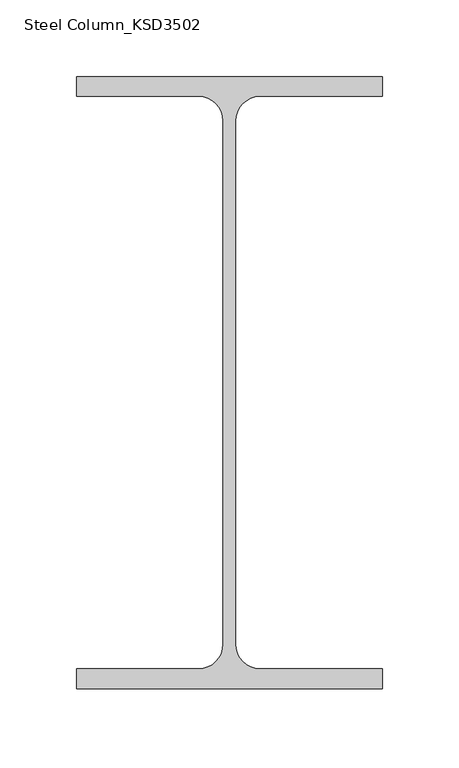
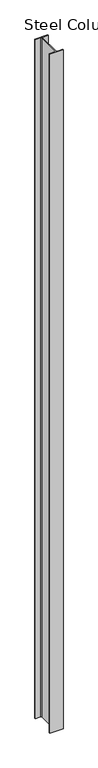
"""IFC4 building model written with IfcOpenShell, lengths in millimetres: column geometry, Steel Column_KSD3502 : H_SC_ASC_H-400×200x8x13."""

import ifcopenshell
import ifcopenshell.guid

model = None  # the IFC model being written
_history = None  # IfcOwnerHistory: only IFC2X3 demands one
_inside = {}  # id of a spatial element -> (the spatial element, [elements in it])
_under = {}  # id of a project, library or spatial element -> (it, [spatial elements below it])
_declared = {}  # id of a project -> (the project, [libraries it declares])
_typed = {}  # id of a type object -> (the type object, [elements of that type])
_made_of = {}  # id of a material, layer set ... -> (it, [elements and type objects made of it])


def new_model(schema):
    """Start an empty IFC model of exactly this schema.

    Asked for "IFC4X3", IfcOpenShell would pick the latest addendum, in which some entities
    have other attributes; the version numbers below select the first issue.
    IFC2X3 requires an IfcOwnerHistory on every rooted entity: one is made here for all.
    """
    global model, _history
    if schema == "IFC4X3":
        model = ifcopenshell.file(schema_version=(4, 3, 0, 0))
    else:
        model = ifcopenshell.file(schema=schema)
    _inside.clear()
    _under.clear()
    _declared.clear()
    _typed.clear()
    _made_of.clear()
    _history = None
    if model.schema == "IFC2X3":
        org = make("IfcOrganization", Name="unknown")
        user = make(
            "IfcPersonAndOrganization",
            ThePerson=make("IfcPerson", FamilyName="unknown"),
            TheOrganization=org,
        )
        app = make(
            "IfcApplication",
            ApplicationDeveloper=org,
            Version="unknown",
            ApplicationFullName="unknown",
            ApplicationIdentifier="unknown",
        )
        _history = make(
            "IfcOwnerHistory",
            OwningUser=user,
            OwningApplication=app,
            ChangeAction="ADDED",
            CreationDate=0,
        )
    return model


def make(cls, **values):
    """One entity of the class cls with the attributes given. An attribute that is None is left unset."""
    return model.create_entity(
        cls, **{name: value for name, value in values.items() if value is not None}
    )


def rooted(cls, **values):
    """An entity with a GlobalId (a new one), such as an element, a storey or a relation."""
    return make(cls, GlobalId=ifcopenshell.guid.new(), OwnerHistory=_history, **values)


def si_unit(unit_type, name, prefix=None):
    """IfcSIUnit, for example si_unit("LENGTHUNIT", "METRE", prefix="MILLI")."""
    return make("IfcSIUnit", UnitType=unit_type, Prefix=prefix, Name=name)


def assignment(units):
    """IfcUnitAssignment: the units of a project."""
    return None if units is None else make("IfcUnitAssignment", Units=units)


def point(xyz):
    """IfcCartesianPoint."""
    return None if xyz is None else make("IfcCartesianPoint", Coordinates=xyz)


def direction(xyz):
    """IfcDirection."""
    return None if xyz is None else make("IfcDirection", DirectionRatios=xyz)


def frame(location, z_axis=None, x_axis=None):
    """IfcAxis2Placement3D, a coordinate frame: its origin and axes. An axis left out is left unset."""
    return make(
        "IfcAxis2Placement3D",
        Location=point(location),
        Axis=direction(z_axis),
        RefDirection=direction(x_axis),
    )


def frame_2d(location, x_axis=None):
    """IfcAxis2Placement2D, a coordinate frame in the plane: its origin and x axis."""
    return make(
        "IfcAxis2Placement2D", Location=point(location), RefDirection=direction(x_axis)
    )


def origin():
    """The frame at (0, 0, 0) with its axes left unset."""
    return frame((0.0, 0.0, 0.0))


def place(relative_to, where):
    """IfcLocalPlacement: puts the frame where relative to a parent placement (None: the world)."""
    return make(
        "IfcLocalPlacement", PlacementRelTo=relative_to, RelativePlacement=where
    )


def context(
    kind, dimensions, precision=None, world=None, true_north=None, identifier=None
):
    """IfcGeometricRepresentationContext, for example the 3D "Model" context."""
    return make(
        "IfcGeometricRepresentationContext",
        ContextIdentifier=identifier,
        ContextType=kind,
        CoordinateSpaceDimension=dimensions,
        Precision=precision,
        WorldCoordinateSystem=world,
        TrueNorth=true_north,
    )


def project(units=None, contexts=None):
    """IfcProject with its units and contexts."""
    return rooted(
        "IfcProject",
        Name="project",
        RepresentationContexts=contexts,
        UnitsInContext=assignment(units),
    )


def spatial(cls, under=None, at=None, **own):
    """A site, building, storey or space (cls), placed at a placement, below another one or the project."""
    s = rooted(cls, ObjectPlacement=at, **own)
    if under is not None:
        _under.setdefault(under.id(), (under, []))[1].append(s)
    return s


def polyline(points):
    """IfcPolyline through the points."""
    return make("IfcPolyline", Points=[point(p) for p in points])


def circle_curve(where, radius):
    """IfcCircle in the frame where."""
    return make("IfcCircle", Position=where, Radius=radius)


def trimmed(basis, trim1, trim2, sense, master):
    """IfcTrimmedCurve: the piece of a basis curve between two trims."""
    return make(
        "IfcTrimmedCurve",
        BasisCurve=basis,
        Trim1=trim1,
        Trim2=trim2,
        SenseAgreement=sense,
        MasterRepresentation=master,
    )


def segment(curve, same_sense, transition):
    """IfcCompositeCurveSegment."""
    return make(
        "IfcCompositeCurveSegment",
        Transition=transition,
        SameSense=same_sense,
        ParentCurve=curve,
    )


def composite_curve(segments, self_intersect=None):
    """IfcCompositeCurve: segments joined end to end."""
    return make("IfcCompositeCurve", Segments=segments, SelfIntersect=self_intersect)


def outline(outer, holes=None, kind="AREA"):
    """IfcArbitraryClosedProfileDef: a profile drawn as a closed curve; with holes, ...WithVoids."""
    if holes is None:
        return make("IfcArbitraryClosedProfileDef", ProfileType=kind, OuterCurve=outer)
    return make(
        "IfcArbitraryProfileDefWithVoids",
        ProfileType=kind,
        OuterCurve=outer,
        InnerCurves=holes,
    )


def extrude(swept, where, along, depth):
    """IfcExtrudedAreaSolid: the profile swept, set in the frame where, extruded along a direction by depth."""
    return make(
        "IfcExtrudedAreaSolid",
        SweptArea=swept,
        Position=where,
        ExtrudedDirection=direction(along),
        Depth=depth,
    )


def shape(context_of_items, identifier, shape_type, items):
    """IfcShapeRepresentation: the items that make up one representation, for example the "Body"."""
    return make(
        "IfcShapeRepresentation",
        ContextOfItems=context_of_items,
        RepresentationIdentifier=identifier,
        RepresentationType=shape_type,
        Items=items,
    )


def source(mapping_origin, context_of_items, identifier, shape_type, items):
    """IfcRepresentationMap: a shape defined once, which mapped items show again and again."""
    return make(
        "IfcRepresentationMap",
        MappingOrigin=mapping_origin,
        MappedRepresentation=shape(context_of_items, identifier, shape_type, items),
    )


def transform(
    local_origin,
    x_axis=None,
    y_axis=None,
    z_axis=None,
    scale=None,
    scale2=None,
    scale3=None,
    uniform=True,
):
    """IfcCartesianTransformationOperator3D, or its non-uniform kind. x_axis, y_axis, z_axis: its Axis1, 2, 3."""
    if uniform:
        return make(
            "IfcCartesianTransformationOperator3D",
            Axis1=direction(x_axis),
            Axis2=direction(y_axis),
            LocalOrigin=point(local_origin),
            Scale=scale,
            Axis3=direction(z_axis),
        )
    return make(
        "IfcCartesianTransformationOperator3DnonUniform",
        Axis1=direction(x_axis),
        Axis2=direction(y_axis),
        LocalOrigin=point(local_origin),
        Scale=scale,
        Axis3=direction(z_axis),
        Scale2=scale2,
        Scale3=scale3,
    )


def mapped(mapping_source, mapping_target):
    """IfcMappedItem: shows the shape of a source again, moved by a transform."""
    return make(
        "IfcMappedItem", MappingSource=mapping_source, MappingTarget=mapping_target
    )


def made_of(thing, what):
    """Note that an element or type object is made of a material, layer set ...; save() writes the relation."""
    if what is not None:
        _made_of.setdefault(what.id(), (what, []))[1].append(thing)
    return thing


def element(
    cls,
    number,
    at=None,
    inside=None,
    cuts=None,
    type_object=None,
    material=None,
    context=None,
    identifier="Body",
    shape_type=None,
    held_by="IfcProductDefinitionShape",
    body=None,
    shapes=None,
    **own,
):
    """One element of the class cls, such as IfcWall. Its Tag is "e" and its number.

    at: its placement. inside: the storey or other place that contains it. cuts: it is an
    opening in that element (IfcRelVoidsElement). A single representation is given by context,
    identifier, shape_type and body (its items); several are given by shapes. held_by: the class
    of the entity that holds the representations. save() writes the other relations.
    """
    e = rooted(cls, Tag="e%d" % number, ObjectPlacement=at, **own)
    if body is not None:
        shapes = [shape(context, identifier, shape_type, body)]
    if shapes is not None:
        e.Representation = make(held_by, Representations=shapes)
    if inside is not None:
        _inside.setdefault(inside.id(), (inside, []))[1].append(e)
    if cuts is not None:
        rooted(
            "IfcRelVoidsElement", RelatingBuildingElement=cuts, RelatedOpeningElement=e
        )
    if type_object is not None:
        _typed.setdefault(type_object.id(), (type_object, []))[1].append(e)
    return made_of(e, material)


def aggregate(whole, parts):
    """IfcRelAggregates: a whole, such as a stair, and the parts it consists of."""
    return rooted("IfcRelAggregates", RelatingObject=whole, RelatedObjects=parts)


def save(model, path):
    """Write the relations noted so far, then the file.

    IfcRelAggregates (storeys below a building ...), IfcRelContainedInSpatialStructure (elements
    in a storey), IfcRelDefinesByType, IfcRelAssociatesMaterial and IfcRelDeclares: one each for
    every whole, place, type object, material and project.
    """
    for whole, parts in _under.values():
        aggregate(whole, parts)
    for where, things in _inside.values():
        rooted(
            "IfcRelContainedInSpatialStructure",
            RelatedElements=things,
            RelatingStructure=where,
        )
    for kind, things in _typed.values():
        rooted("IfcRelDefinesByType", RelatedObjects=things, RelatingType=kind)
    for what, things in _made_of.values():
        rooted("IfcRelAssociatesMaterial", RelatedObjects=things, RelatingMaterial=what)
    for by, libraries in _declared.values():
        rooted("IfcRelDeclares", RelatingContext=by, RelatedDefinitions=libraries)
    model.write(path)


def steel_column_ksd3502_a45a25b2(model_context):
    return source(origin(), model_context, "Body", "SweptSolid", [
        extrude(outline(composite_curve([segment(polyline([(100.0, 200.0), (100.0, 187.0), (20.0, 187.0)]), True, "CONTINUOUS"), segment(trimmed(circle_curve(frame_2d((20.0, 171.0)), 16.0), [point((20.0, 187.0))], [point((4.0, 171.0))], True, "CARTESIAN"), True, "CONTINUOUS"), segment(polyline([(4.0, 171.0), (4.0, -171.0)]), True, "CONTINUOUS"), segment(trimmed(circle_curve(frame_2d((20.0, -171.0)), 16.0), [point((4.0, -171.0))], [point((20.0, -187.0))], True, "CARTESIAN"), True, "CONTINUOUS"), segment(polyline([(20.0, -187.0), (100.0, -187.0), (100.0, -200.0), (-100.0, -200.0), (-100.0, -187.0), (-20.0, -187.0)]), True, "CONTINUOUS"), segment(trimmed(circle_curve(frame_2d((-20.0, -171.0)), 16.0), [point((-20.0, -187.0))], [point((-4.0, -171.0))], True, "CARTESIAN"), True, "CONTINUOUS"), segment(polyline([(-4.0, -171.0), (-4.0, 171.0)]), True, "CONTINUOUS"), segment(trimmed(circle_curve(frame_2d((-20.0, 171.0)), 16.0), [point((-4.0, 171.0))], [point((-20.0, 187.0))], True, "CARTESIAN"), True, "CONTINUOUS"), segment(polyline([(-20.0, 187.0), (-100.0, 187.0), (-100.0, 200.0), (100.0, 200.0)]), True, "CONTINUOUS")], self_intersect=False)), frame((0.0, 0.0, 6649.9720055), z_axis=(0.0, 0.0, 1.0), x_axis=(1.0, 0.0, 0.0)), (0.0, 0.0, 1.0), 11000.0),
    ])


if __name__ == "__main__":
    model = new_model("IFC4")
    model_context = context("Model", 3, world=origin())
    ifc_project = project(units=[si_unit("LENGTHUNIT", "METRE", prefix="MILLI")], contexts=[model_context])
    site = spatial("IfcSite", under=ifc_project)
    building = spatial("IfcBuilding", under=site)
    placement = place(None, origin())
    steel_column_ksd3502_shape = steel_column_ksd3502_a45a25b2(model_context)
    element("IfcColumn", 1, ObjectType="Steel Column_KSD3502 : H_SC_ASC_H-400×200x8x13", at=placement, inside=building, context=model_context, shape_type="MappedRepresentation", body=[
        mapped(steel_column_ksd3502_shape, transform((0.0, 0.0, 0.0), x_axis=(1.0, 0.0, 0.0), y_axis=(0.0, 1.0, 0.0), z_axis=(0.0, 0.0, 1.0))),
    ])
    save(model, "model.ifc")

# Revit data of these elements
# Type "Steel Column_KSD3502 : H_SC_ASC_H-400×200x8x13"
#   Width = 20.0 cm
#   Web Thickness = 0.8 cm
#   Web Fillet = 1.6 cm
#   Warping Constant = 648999.0 cm⁶
#   Torsional Moment of Inertia = 35.8981 cm⁴
#   Section Area = 84.12 cm²
#   Plastic Modulus weak axis = 268.0 cm³
#   Plastic Modulus strong axis = 1330.0 cm³
#   Perimeter = 1.27 m²/m
#   Nominal Weight = 66.00 kgf/m
#   Moment of Inertia weak axis = 1740.00 cm⁴
#   Moment of Inertia strong axis = 23700.00 cm⁴
#   Height = 40.0 cm
#   Flange Thickness = 1.3 cm
#   Elastic Modulus weak axis = 174.0 cm³
#   Elastic Modulus strong axis = 1190.0 cm³
#   Centroid Vertical = 20.0 cm
#   Centroid Horizontal = 10.0 cm
#   Bolt Spacing = 13.97 cm
#   Structural Material [instance default] = Steel, 45-345
#   Section Name Key = ""
#   Assembly Code = ""
# Element 1 (IfcColumn, "Steel Column_KSD3502 : H_SC_ASC_H-400×200x8x13")
#   Structural Material = none
# Materials
#   "Steel, 45-345": class "Metal", colour RGB 189 187 185, transparency 0, Description = "Steel 345 MPa", Cost = 0
